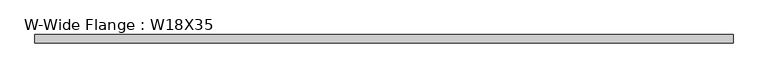
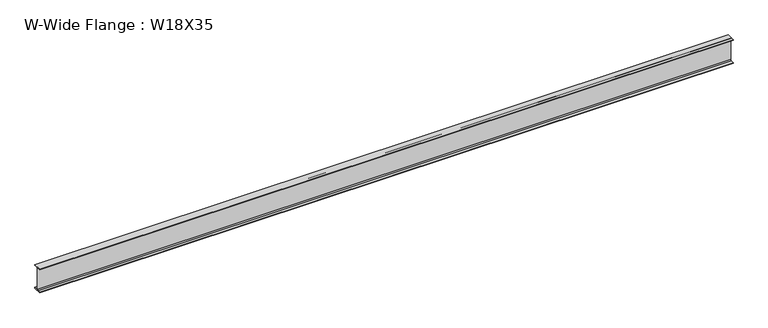
"""IFC4 building model written with IfcOpenShell, lengths in millimetres: beam geometry, W-Wide Flange : W18X35."""

import ifcopenshell
import ifcopenshell.guid

model = None  # the IFC model being written
_history = None  # IfcOwnerHistory: only IFC2X3 demands one
_inside = {}  # id of a spatial element -> (the spatial element, [elements in it])
_under = {}  # id of a project, library or spatial element -> (it, [spatial elements below it])
_declared = {}  # id of a project -> (the project, [libraries it declares])
_typed = {}  # id of a type object -> (the type object, [elements of that type])
_made_of = {}  # id of a material, layer set ... -> (it, [elements and type objects made of it])


def new_model(schema):
    """Start an empty IFC model of exactly this schema.

    Asked for "IFC4X3", IfcOpenShell would pick the latest addendum, in which some entities
    have other attributes; the version numbers below select the first issue.
    IFC2X3 requires an IfcOwnerHistory on every rooted entity: one is made here for all.
    """
    global model, _history
    if schema == "IFC4X3":
        model = ifcopenshell.file(schema_version=(4, 3, 0, 0))
    else:
        model = ifcopenshell.file(schema=schema)
    _inside.clear()
    _under.clear()
    _declared.clear()
    _typed.clear()
    _made_of.clear()
    _history = None
    if model.schema == "IFC2X3":
        org = make("IfcOrganization", Name="unknown")
        user = make(
            "IfcPersonAndOrganization",
            ThePerson=make("IfcPerson", FamilyName="unknown"),
            TheOrganization=org,
        )
        app = make(
            "IfcApplication",
            ApplicationDeveloper=org,
            Version="unknown",
            ApplicationFullName="unknown",
            ApplicationIdentifier="unknown",
        )
        _history = make(
            "IfcOwnerHistory",
            OwningUser=user,
            OwningApplication=app,
            ChangeAction="ADDED",
            CreationDate=0,
        )
    return model


def make(cls, **values):
    """One entity of the class cls with the attributes given. An attribute that is None is left unset."""
    return model.create_entity(
        cls, **{name: value for name, value in values.items() if value is not None}
    )


def rooted(cls, **values):
    """An entity with a GlobalId (a new one), such as an element, a storey or a relation."""
    return make(cls, GlobalId=ifcopenshell.guid.new(), OwnerHistory=_history, **values)


def si_unit(unit_type, name, prefix=None):
    """IfcSIUnit, for example si_unit("LENGTHUNIT", "METRE", prefix="MILLI")."""
    return make("IfcSIUnit", UnitType=unit_type, Prefix=prefix, Name=name)


def assignment(units):
    """IfcUnitAssignment: the units of a project."""
    return None if units is None else make("IfcUnitAssignment", Units=units)


def point(xyz):
    """IfcCartesianPoint."""
    return None if xyz is None else make("IfcCartesianPoint", Coordinates=xyz)


def direction(xyz):
    """IfcDirection."""
    return None if xyz is None else make("IfcDirection", DirectionRatios=xyz)


def frame(location, z_axis=None, x_axis=None):
    """IfcAxis2Placement3D, a coordinate frame: its origin and axes. An axis left out is left unset."""
    return make(
        "IfcAxis2Placement3D",
        Location=point(location),
        Axis=direction(z_axis),
        RefDirection=direction(x_axis),
    )


def frame_2d(location, x_axis=None):
    """IfcAxis2Placement2D, a coordinate frame in the plane: its origin and x axis."""
    return make(
        "IfcAxis2Placement2D", Location=point(location), RefDirection=direction(x_axis)
    )


def origin():
    """The frame at (0, 0, 0) with its axes left unset."""
    return frame((0.0, 0.0, 0.0))


def place(relative_to, where):
    """IfcLocalPlacement: puts the frame where relative to a parent placement (None: the world)."""
    return make(
        "IfcLocalPlacement", PlacementRelTo=relative_to, RelativePlacement=where
    )


def context(
    kind, dimensions, precision=None, world=None, true_north=None, identifier=None
):
    """IfcGeometricRepresentationContext, for example the 3D "Model" context."""
    return make(
        "IfcGeometricRepresentationContext",
        ContextIdentifier=identifier,
        ContextType=kind,
        CoordinateSpaceDimension=dimensions,
        Precision=precision,
        WorldCoordinateSystem=world,
        TrueNorth=true_north,
    )


def project(units=None, contexts=None):
    """IfcProject with its units and contexts."""
    return rooted(
        "IfcProject",
        Name="project",
        RepresentationContexts=contexts,
        UnitsInContext=assignment(units),
    )


def spatial(cls, under=None, at=None, **own):
    """A site, building, storey or space (cls), placed at a placement, below another one or the project."""
    s = rooted(cls, ObjectPlacement=at, **own)
    if under is not None:
        _under.setdefault(under.id(), (under, []))[1].append(s)
    return s


def polyline(points):
    """IfcPolyline through the points."""
    return make("IfcPolyline", Points=[point(p) for p in points])


def circle_curve(where, radius):
    """IfcCircle in the frame where."""
    return make("IfcCircle", Position=where, Radius=radius)


def trimmed(basis, trim1, trim2, sense, master):
    """IfcTrimmedCurve: the piece of a basis curve between two trims."""
    return make(
        "IfcTrimmedCurve",
        BasisCurve=basis,
        Trim1=trim1,
        Trim2=trim2,
        SenseAgreement=sense,
        MasterRepresentation=master,
    )


def segment(curve, same_sense, transition):
    """IfcCompositeCurveSegment."""
    return make(
        "IfcCompositeCurveSegment",
        Transition=transition,
        SameSense=same_sense,
        ParentCurve=curve,
    )


def composite_curve(segments, self_intersect=None):
    """IfcCompositeCurve: segments joined end to end."""
    return make("IfcCompositeCurve", Segments=segments, SelfIntersect=self_intersect)


def outline(outer, holes=None, kind="AREA"):
    """IfcArbitraryClosedProfileDef: a profile drawn as a closed curve; with holes, ...WithVoids."""
    if holes is None:
        return make("IfcArbitraryClosedProfileDef", ProfileType=kind, OuterCurve=outer)
    return make(
        "IfcArbitraryProfileDefWithVoids",
        ProfileType=kind,
        OuterCurve=outer,
        InnerCurves=holes,
    )


def extrude(swept, where, along, depth):
    """IfcExtrudedAreaSolid: the profile swept, set in the frame where, extruded along a direction by depth."""
    return make(
        "IfcExtrudedAreaSolid",
        SweptArea=swept,
        Position=where,
        ExtrudedDirection=direction(along),
        Depth=depth,
    )


def shape(context_of_items, identifier, shape_type, items):
    """IfcShapeRepresentation: the items that make up one representation, for example the "Body"."""
    return make(
        "IfcShapeRepresentation",
        ContextOfItems=context_of_items,
        RepresentationIdentifier=identifier,
        RepresentationType=shape_type,
        Items=items,
    )


def source(mapping_origin, context_of_items, identifier, shape_type, items):
    """IfcRepresentationMap: a shape defined once, which mapped items show again and again."""
    return make(
        "IfcRepresentationMap",
        MappingOrigin=mapping_origin,
        MappedRepresentation=shape(context_of_items, identifier, shape_type, items),
    )


def transform(
    local_origin,
    x_axis=None,
    y_axis=None,
    z_axis=None,
    scale=None,
    scale2=None,
    scale3=None,
    uniform=True,
):
    """IfcCartesianTransformationOperator3D, or its non-uniform kind. x_axis, y_axis, z_axis: its Axis1, 2, 3."""
    if uniform:
        return make(
            "IfcCartesianTransformationOperator3D",
            Axis1=direction(x_axis),
            Axis2=direction(y_axis),
            LocalOrigin=point(local_origin),
            Scale=scale,
            Axis3=direction(z_axis),
        )
    return make(
        "IfcCartesianTransformationOperator3DnonUniform",
        Axis1=direction(x_axis),
        Axis2=direction(y_axis),
        LocalOrigin=point(local_origin),
        Scale=scale,
        Axis3=direction(z_axis),
        Scale2=scale2,
        Scale3=scale3,
    )


def mapped(mapping_source, mapping_target):
    """IfcMappedItem: shows the shape of a source again, moved by a transform."""
    return make(
        "IfcMappedItem", MappingSource=mapping_source, MappingTarget=mapping_target
    )


def made_of(thing, what):
    """Note that an element or type object is made of a material, layer set ...; save() writes the relation."""
    if what is not None:
        _made_of.setdefault(what.id(), (what, []))[1].append(thing)
    return thing


def element(
    cls,
    number,
    at=None,
    inside=None,
    cuts=None,
    type_object=None,
    material=None,
    context=None,
    identifier="Body",
    shape_type=None,
    held_by="IfcProductDefinitionShape",
    body=None,
    shapes=None,
    **own,
):
    """One element of the class cls, such as IfcWall. Its Tag is "e" and its number.

    at: its placement. inside: the storey or other place that contains it. cuts: it is an
    opening in that element (IfcRelVoidsElement). A single representation is given by context,
    identifier, shape_type and body (its items); several are given by shapes. held_by: the class
    of the entity that holds the representations. save() writes the other relations.
    """
    e = rooted(cls, Tag="e%d" % number, ObjectPlacement=at, **own)
    if body is not None:
        shapes = [shape(context, identifier, shape_type, body)]
    if shapes is not None:
        e.Representation = make(held_by, Representations=shapes)
    if inside is not None:
        _inside.setdefault(inside.id(), (inside, []))[1].append(e)
    if cuts is not None:
        rooted(
            "IfcRelVoidsElement", RelatingBuildingElement=cuts, RelatedOpeningElement=e
        )
    if type_object is not None:
        _typed.setdefault(type_object.id(), (type_object, []))[1].append(e)
    return made_of(e, material)


def aggregate(whole, parts):
    """IfcRelAggregates: a whole, such as a stair, and the parts it consists of."""
    return rooted("IfcRelAggregates", RelatingObject=whole, RelatedObjects=parts)


def save(model, path):
    """Write the relations noted so far, then the file.

    IfcRelAggregates (storeys below a building ...), IfcRelContainedInSpatialStructure (elements
    in a storey), IfcRelDefinesByType, IfcRelAssociatesMaterial and IfcRelDeclares: one each for
    every whole, place, type object, material and project.
    """
    for whole, parts in _under.values():
        aggregate(whole, parts)
    for where, things in _inside.values():
        rooted(
            "IfcRelContainedInSpatialStructure",
            RelatedElements=things,
            RelatingStructure=where,
        )
    for kind, things in _typed.values():
        rooted("IfcRelDefinesByType", RelatedObjects=things, RelatingType=kind)
    for what, things in _made_of.values():
        rooted("IfcRelAssociatesMaterial", RelatedObjects=things, RelatingMaterial=what)
    for by, libraries in _declared.values():
        rooted("IfcRelDeclares", RelatingContext=by, RelatedDefinitions=libraries)
    model.write(path)


def w_wide_flange_w18x35_dd771225(model_context):
    return source(origin(), model_context, "Body", "SweptSolid", [
        extrude(outline(composite_curve([segment(polyline([(76.2, -213.995), (76.2, -224.79), (-76.2, -224.79), (-76.2, -213.995), (-21.59, -213.995)]), True, "CONTINUOUS"), segment(trimmed(circle_curve(frame_2d((-21.59, -196.215)), 17.78), [point((-21.59, -213.995))], [point((-3.81, -196.215))], True, "CARTESIAN"), True, "CONTINUOUS"), segment(polyline([(-3.81, -196.215), (-3.81, 196.215)]), True, "CONTINUOUS"), segment(trimmed(circle_curve(frame_2d((-21.59, 196.215)), 17.78), [point((-3.81, 196.215))], [point((-21.59, 213.995))], True, "CARTESIAN"), True, "CONTINUOUS"), segment(polyline([(-21.59, 213.995), (-76.2, 213.995), (-76.2, 224.79), (76.2, 224.79), (76.2, 213.995), (21.59, 213.995)]), True, "CONTINUOUS"), segment(trimmed(circle_curve(frame_2d((21.59, 196.215)), 17.78), [point((21.59, 213.995))], [point((3.81, 196.215))], True, "CARTESIAN"), True, "CONTINUOUS"), segment(polyline([(3.81, 196.215), (3.81, -196.215)]), True, "CONTINUOUS"), segment(trimmed(circle_curve(frame_2d((21.59, -196.215)), 17.78), [point((3.81, -196.215))], [point((21.59, -213.995))], True, "CARTESIAN"), True, "CONTINUOUS"), segment(polyline([(21.59, -213.995), (76.2, -213.995)]), True, "CONTINUOUS")], self_intersect=False)), frame((-6252.7104992, 0.0, 0.0), z_axis=(1.0, 0.0, 0.0), x_axis=(0.0, 1.0, 0.0)), (0.0, 0.0, 1.0), 12523.1165167),
    ])


if __name__ == "__main__":
    model = new_model("IFC4")
    model_context = context("Model", 3, world=origin())
    ifc_project = project(units=[si_unit("LENGTHUNIT", "METRE", prefix="MILLI")], contexts=[model_context])
    site = spatial("IfcSite", under=ifc_project)
    building = spatial("IfcBuilding", under=site)
    placement = place(None, origin())
    w_wide_flange_w18x35_shape = w_wide_flange_w18x35_dd771225(model_context)
    element("IfcBeam", 1, ObjectType="W-Wide Flange : W18X35", at=placement, inside=building, context=model_context, shape_type="MappedRepresentation", body=[
        mapped(w_wide_flange_w18x35_shape, transform((0.0, 0.0, 0.0), x_axis=(1.0, 0.0, 0.0), y_axis=(0.0, 1.0, 0.0), z_axis=(0.0, 0.0, 1.0))),
    ])
    save(model, "model.ifc")

# Revit data of these elements
# Type "W-Wide Flange : W18X35"
#   Assembly Code = "B10"
#   W = 35
#   Length [instance default] = 5' - 0"
#   bf = 0' - 6"
#   d = 1' - 5.7"
#   k = 0' - 1 1/8"
#   k2 = 0' - 0.7"
#   tf = 0' - 0.425"
#   tw = 0' - 0.3"
#   A = 0.0715278 SF
#   Structural Material [instance default] = Steel ASTM A992
# Element 1 (IfcBeam, "W-Wide Flange : W18X35")
#   Structural Material = Steel ASTM A36
#   Materials on its faces: "Steel ASTM A36"
# Materials
#   "Steel ASTM A992": class "Metal", colour RGB 199 199 199, transparency 0, Description = "Structural steel 50ksi", Cost = 0
#   "Steel ASTM A36": class "Metal", colour RGB 199 199 199, transparency 0, Description = "Structural steel, ASTM A36 Grade B, mill finish", Cost = 0
